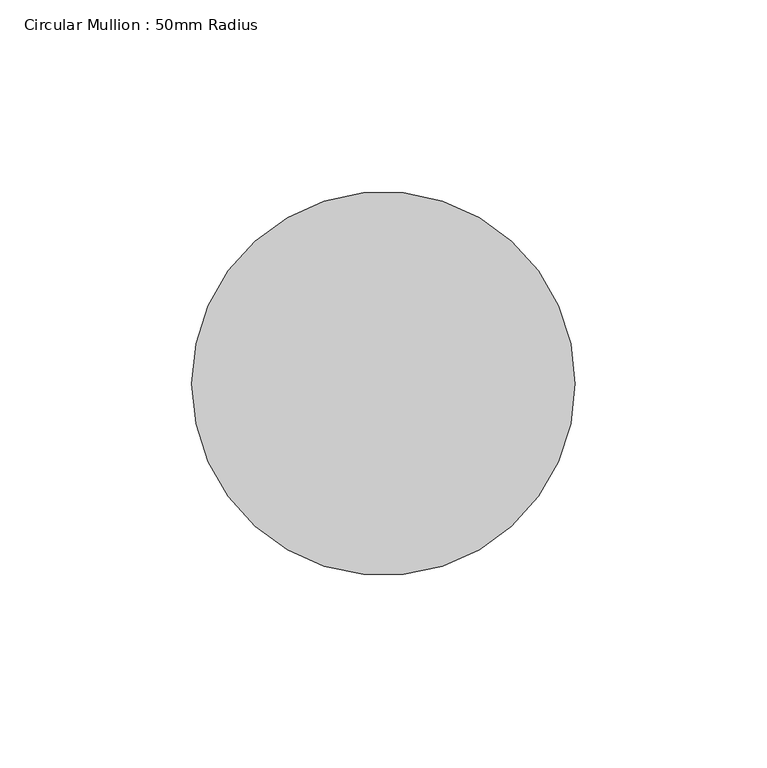
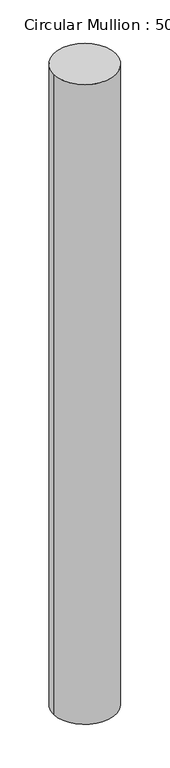
"""IFC4 building model written with IfcOpenShell, lengths in millimetres: member geometry, Circular Mullion : 50mm Radius."""

from ifc_helpers import new_model, si_unit, point, frame, origin, origin_2d, place, context, project, spatial, circle_curve, trimmed, segment, composite_curve, outline, extrude, source, transform, mapped, element, save


def circular_mullion_50mm_radius_07812386(model_context):
    return source(origin(), model_context, "Body", "SweptSolid", [
        extrude(outline(composite_curve([segment(trimmed(circle_curve(origin_2d(), 50.0), [point((50.0, 0.0))], [point((-50.0, 0.0))], False, "CARTESIAN"), True, "CONTINUOUS"), segment(trimmed(circle_curve(origin_2d(), 50.0), [point((-50.0, 0.0))], [point((50.0, 0.0))], False, "CARTESIAN"), True, "CONTINUOUS")], self_intersect=False)), frame((0.0, 0.0, -1086.9588947), z_axis=(0.0, 0.0, 1.0), x_axis=(1.0, 0.0, 0.0)), (0.0, 0.0, 1.0), 1086.9588947),
    ])


if __name__ == "__main__":
    model = new_model("IFC4")
    model_context = context("Model", 3, world=origin())
    ifc_project = project(units=[si_unit("LENGTHUNIT", "METRE", prefix="MILLI")], contexts=[model_context])
    site = spatial("IfcSite", under=ifc_project)
    building = spatial("IfcBuilding", under=site)
    placement = place(None, origin())
    circular_mullion_50mm_radius_shape = circular_mullion_50mm_radius_07812386(model_context)
    element("IfcMember", 1, ObjectType="Circular Mullion : 50mm Radius", at=placement, inside=building, context=model_context, shape_type="MappedRepresentation", body=[
        mapped(circular_mullion_50mm_radius_shape, transform((0.0, 0.0, 0.0), x_axis=(1.0, 0.0, 0.0), y_axis=(0.0, 1.0, 0.0), z_axis=(0.0, 0.0, 1.0))),
    ])
    save(model, "model.ifc")

# Revit data of these elements
# Type "Circular Mullion : 50mm Radius"
#   built-in parameter 1007350 = 0.164042 (stored number, unit not read)
# Element 1 (IfcMember, "Circular Mullion : 50mm Radius")
#   Materials on its faces: "Aluminium"
# Materials
#   "Aluminium": class "Metal", colour RGB 247 247 247, transparency 0, Description = "Aluminium 6061", Cost = 0
